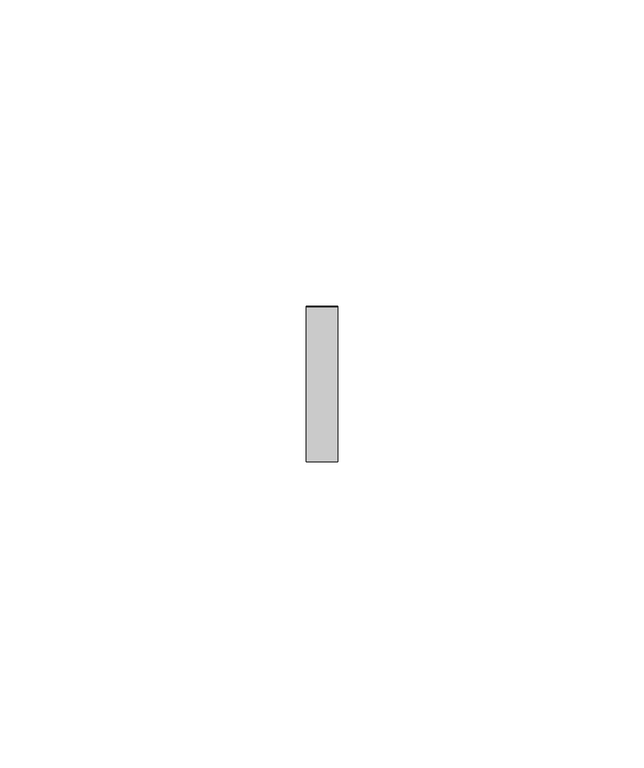
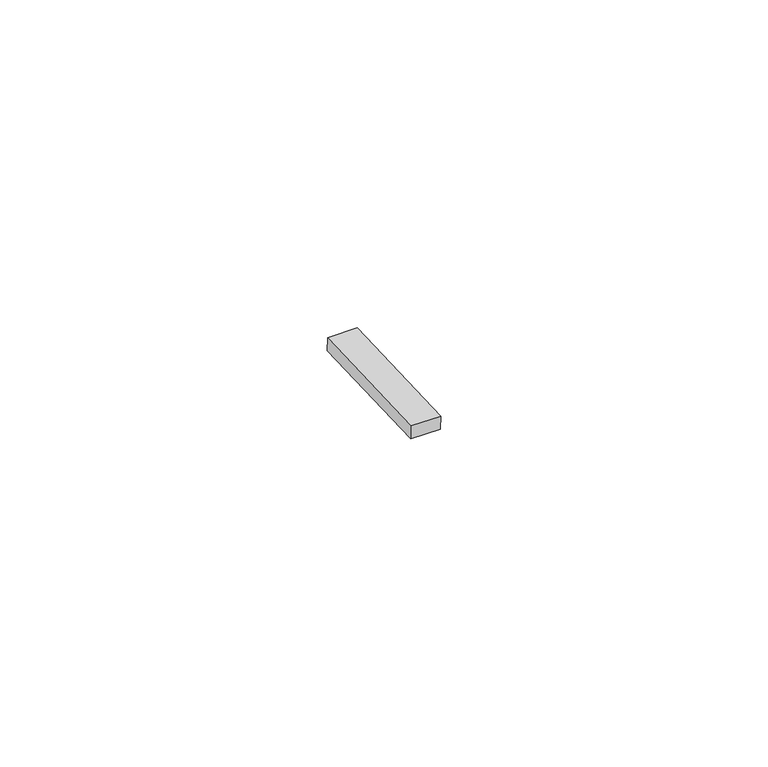
"""IFC4 building model written with IfcOpenShell, lengths in millimetres: proxy geometry, Inner panel:Inner panel:1:Inner panel:1 : Inner panel:Inner panel:300324:2:Inner panel:1:Inner panel:1 : Inner panel:Inner panel:300324:2 : Inner panel:Inner panel:1:Inner panel:1 : Inner panel:Inner panel:300324:300043:129 : Inner panel:Inner panel:1:Inner panel:1 : Inner panel:Inner panel:300324:2:Inner panel:1:Inner panel:1 : Inner panel:Inner panel:300324:2 : Inner panel:Inner panel:1:Inner panel:1 : Inner panel:Inner panel:300324:300043:308120."""

from ifc_helpers import new_model, si_unit, frame, origin, place, context, project, spatial, polyline, outline, extrude, source, transform, mapped, element, save


def generic_models_7856574d(model_context):
    return source(origin(), model_context, "Body", "SweptSolid", [
        extrude(outline(polyline([(0.0, -25.3999999), (0.0, 0.0), (5.2138089, 0.0), (5.2138089, -25.3999999), (0.0, -25.3999999)])), frame((591904.595117, -577413.7950993, 4016.01903), z_axis=(0.0, -0.041630544712223896, 0.9991330730923502), x_axis=(-1.0, 0.0, 0.0)), (0.0, 0.0, 1.0), 2.4763745),
    ])


if __name__ == "__main__":
    model = new_model("IFC4")
    model_context = context("Model", 3, world=origin())
    ifc_project = project(units=[si_unit("LENGTHUNIT", "METRE", prefix="MILLI")], contexts=[model_context])
    site = spatial("IfcSite", under=ifc_project)
    building = spatial("IfcBuilding", under=site)
    placement = place(None, origin())
    generic_models_shape = generic_models_7856574d(model_context)
    element("IfcBuildingElementProxy", 1, Name="Inner panel:Inner panel:1:Inner panel:1 : Inner panel:Inner panel:300324:2:Inner panel:1:Inner panel:1 : Inner panel:Inner panel:300324:2 : Inner panel:Inner panel:1:Inner panel:1 : Inner panel:Inner panel:300324:300043:129 : Inner panel:Inner panel:1:Inner panel:1 : Inner panel:Inner panel:300324:2:Inner panel:1:Inner panel:1 : Inner panel:Inner panel:300324:2 : Inner panel:Inner panel:1:Inner panel:1 : Inner panel:Inner panel:300324:300043:308120", ObjectType="Inner panel:Inner panel:1:Inner panel:1 : Inner panel:Inner panel:300324:2:Inner panel:1:Inner panel:1 : Inner panel:Inner panel:300324:2 : Inner panel:Inner panel:1:Inner panel:1 : Inner panel:Inner panel:300324:300043:129 : Inner panel:Inner panel:1:Inner panel:1 : Inner panel:Inner panel:300324:2:Inner panel:1:Inner panel:1 : Inner panel:Inner panel:300324:2 : Inner panel:Inner panel:1:Inner panel:1 : Inner panel:Inner panel:300324:300043:308120", at=placement, inside=building, context=model_context, shape_type="MappedRepresentation", body=[
        mapped(generic_models_shape, transform((0.0, 0.0, 0.0), x_axis=(1.0, 0.0, 0.0), y_axis=(0.0, 1.0, 0.0), z_axis=(0.0, 0.0, 1.0))),
    ])
    save(model, "model.ifc")

# Revit data of these elements
# Type "Inner panel:Inner panel:1:Inner panel:1 : Inner panel:Inner panel:300324:2:Inner panel:1:Inner panel:1 : Inner panel:Inner panel:300324:2 : Inner panel:Inner panel:1:Inner panel:1 : Inner panel:Inner panel:300324:300043:129 : Inner panel:Inner panel:1:Inner panel:1 : Inner panel:Inner panel:300324:2:Inner panel:1:Inner panel:1 : Inner panel:Inner panel:300324:2 : Inner panel:Inner panel:1:Inner panel:1 : Inner panel:Inner panel:300324:300043:308120"
#   NameOverride = "Inner panel:Inner panel:1:Inner panel:1 : Inner panel:Inner panel:300324:2:Inner panel:1:Inner panel:1 : Inner panel:Inner panel:300324:2 : Inner panel:Inner panel:1:Inner panel:1 : Inner panel:Inner panel:300324:300043:308120"
#   ObjectTypeOverride = "Inner panel:1:Inner panel:1 : Inner panel:Inner panel:300324:2 : Inner panel:Inner panel:1:Inner panel:1 : Inner panel:Inner panel:300324:300043"
#   Reference = "Inner panel"
#   Tag = "308120"
# Element 1 (IfcBuildingElementProxy, "Inner panel:Inner panel:1:Inner panel:1 : Inner panel:Inner panel:300324:2:Inner panel:1:Inner panel:1 : Inner panel:Inner panel:300324:2 : Inner panel:Inner panel:1:Inner panel:1 : Inner panel:Inner panel:300324:300043:129 : Inner panel:Inner panel:1:Inner panel:1 : Inner panel:Inner panel:300324:2:Inner panel:1:Inner panel:1 : Inner panel:Inner panel:300324:2 : Inner panel:Inner panel:1:Inner panel:1 : Inner panel:Inner panel:300324:300043:308120")
#   Materials on its faces: "AT CLIP - 1\" WIDE NON ABSORBENT, WEATHER-RESISTANT NEOPRENE/EPDM/SBR FOAM"
# Materials
#   "AT CLIP - 1\" WIDE NON ABSORBENT, WEATHER-RESISTANT NEOPRENE/EPDM/SBR FOAM": class "Generic", colour RGB 85 85 85, transparency 0, Cost = 0
